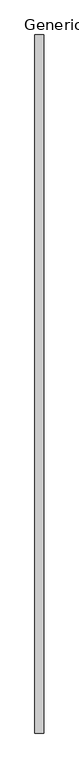
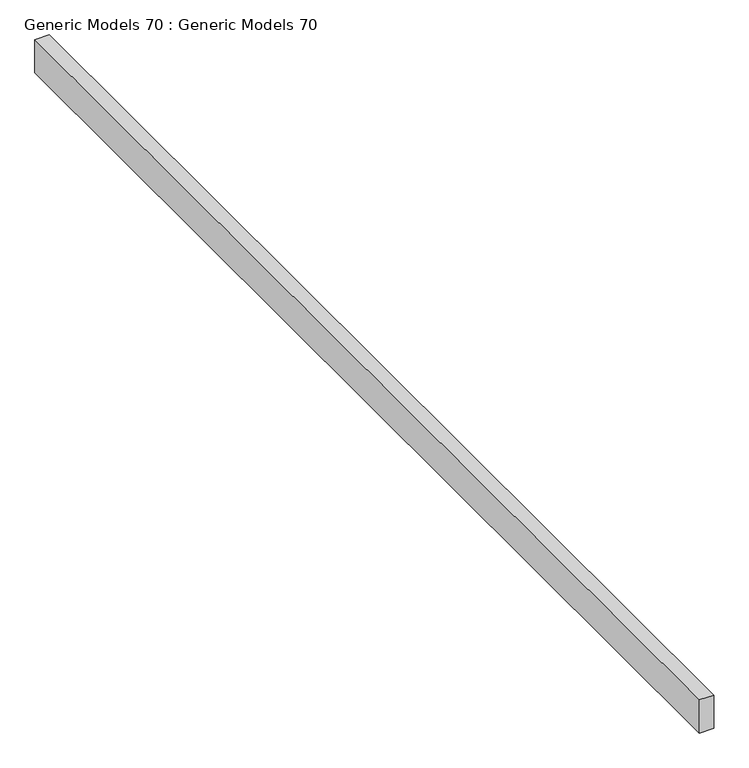
"""IFC4 building model written with IfcOpenShell, lengths in millimetres: proxy geometry, Generic Models 70 : Generic Models 70."""

from ifc_helpers import new_model, si_unit, frame, origin, place, context, project, spatial, polyline, outline, extrude, source, transform, mapped, element, save


def generic_models_70_generic_models_70_98601c22(model_context):
    return source(origin(), model_context, "Body", "SweptSolid", [
        extrude(outline(polyline([(31923.0340778, 39663.9958903), (31923.0340778, 28437.6872112), (31783.3340778, 28437.6872112), (31783.3340778, 39663.9958903), (31923.0340778, 39663.9958903)])), frame((0.0, 0.0, 271462.5), z_axis=(0.0, 0.0, 1.0), x_axis=(1.0, 0.0, 0.0)), (0.0, 0.0, 1.0), 342.9),
    ])


if __name__ == "__main__":
    model = new_model("IFC4")
    model_context = context("Model", 3, world=origin())
    ifc_project = project(units=[si_unit("LENGTHUNIT", "METRE", prefix="MILLI")], contexts=[model_context])
    site = spatial("IfcSite", under=ifc_project)
    building = spatial("IfcBuilding", under=site)
    placement = place(None, origin())
    generic_models_70_generic_models_70_shape = generic_models_70_generic_models_70_98601c22(model_context)
    element("IfcBuildingElementProxy", 1, Name="Generic Models 70 : Generic Models 70", ObjectType="Generic Models 70 : Generic Models 70", at=placement, inside=building, context=model_context, shape_type="MappedRepresentation", body=[
        mapped(generic_models_70_generic_models_70_shape, transform((0.0, 0.0, 0.0), x_axis=(1.0, 0.0, 0.0), y_axis=(0.0, 1.0, 0.0), z_axis=(0.0, 0.0, 1.0))),
    ])
    save(model, "model.ifc")

# Revit data of these elements
# Element 1 (IfcBuildingElementProxy, "Generic Models 70 : Generic Models 70")
#   Materials on its faces: "5 1/2\" x 13 1/2\" GLUELAM BEAM"
# Materials
#   "5 1/2\" x 13 1/2\" GLUELAM BEAM": class "Wood", colour RGB 211 164 143, transparency 0, Description = "Pinus Echinata", Cost = 0
